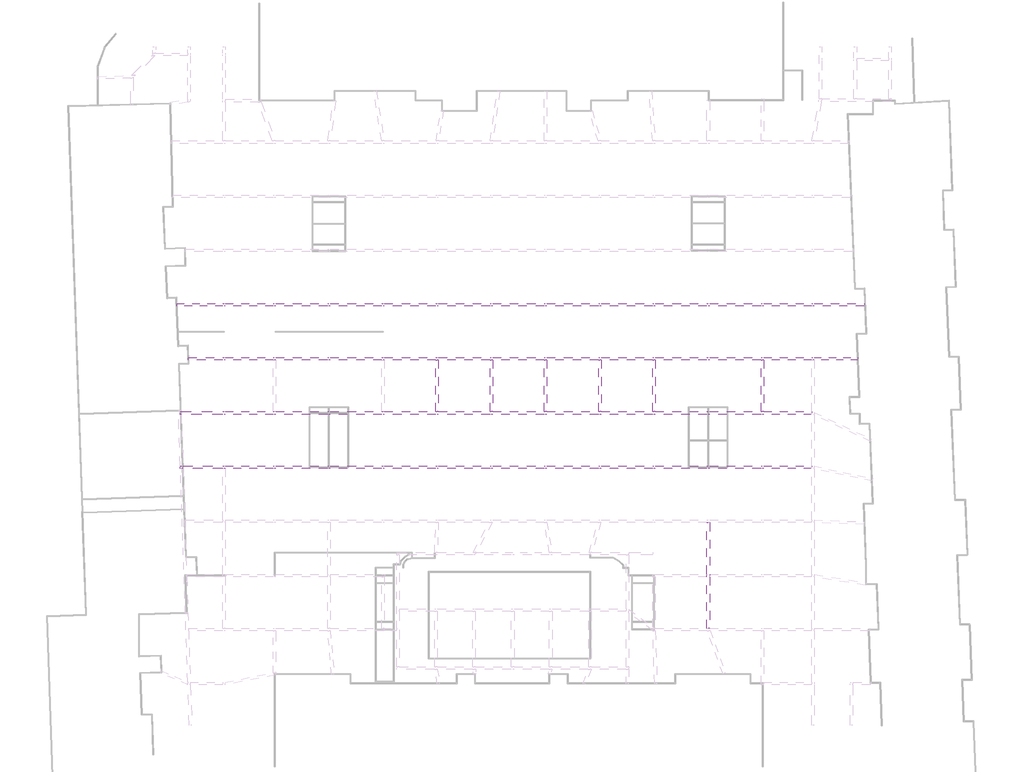
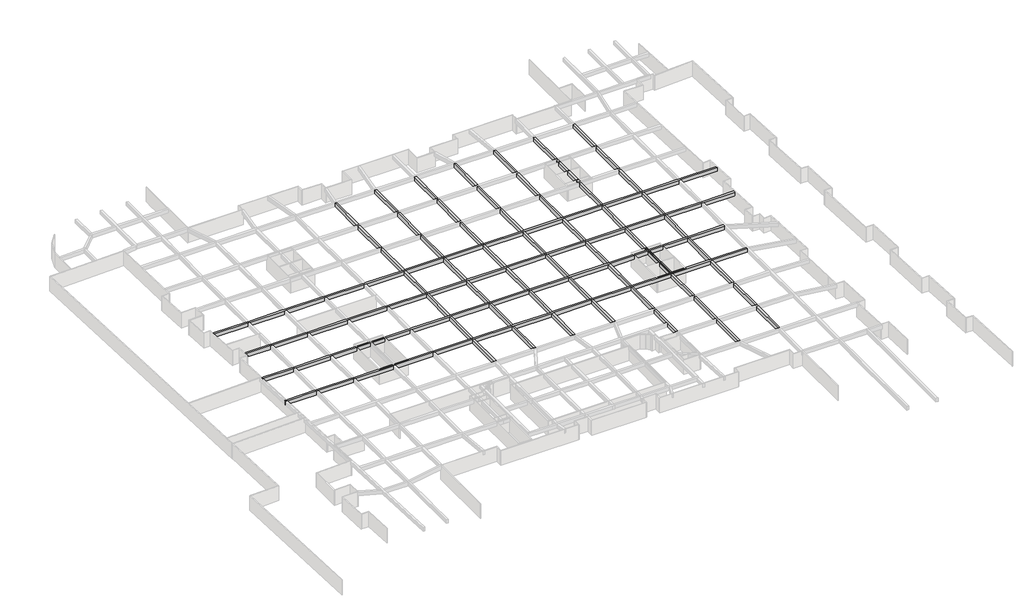
# One storey, part 7 of 8: 11 beams.
"""IFC4 building model written with IfcOpenShell, lengths in millimetres."""

import ifcopenshell
import ifcopenshell.guid

model = None  # the IFC model being written
_history = None  # IfcOwnerHistory: only IFC2X3 demands one
_inside = {}  # id of a spatial element -> (the spatial element, [elements in it])
_under = {}  # id of a project, library or spatial element -> (it, [spatial elements below it])
_declared = {}  # id of a project -> (the project, [libraries it declares])
_typed = {}  # id of a type object -> (the type object, [elements of that type])
_made_of = {}  # id of a material, layer set ... -> (it, [elements and type objects made of it])


def new_model(schema):
    """Start an empty IFC model of exactly this schema.

    Asked for "IFC4X3", IfcOpenShell would pick the latest addendum, in which some entities
    have other attributes; the version numbers below select the first issue.
    IFC2X3 requires an IfcOwnerHistory on every rooted entity: one is made here for all.
    """
    global model, _history
    if schema == "IFC4X3":
        model = ifcopenshell.file(schema_version=(4, 3, 0, 0))
    else:
        model = ifcopenshell.file(schema=schema)
    _inside.clear()
    _under.clear()
    _declared.clear()
    _typed.clear()
    _made_of.clear()
    _history = None
    if model.schema == "IFC2X3":
        org = make("IfcOrganization", Name="unknown")
        user = make(
            "IfcPersonAndOrganization",
            ThePerson=make("IfcPerson", FamilyName="unknown"),
            TheOrganization=org,
        )
        app = make(
            "IfcApplication",
            ApplicationDeveloper=org,
            Version="unknown",
            ApplicationFullName="unknown",
            ApplicationIdentifier="unknown",
        )
        _history = make(
            "IfcOwnerHistory",
            OwningUser=user,
            OwningApplication=app,
            ChangeAction="ADDED",
            CreationDate=0,
        )
    return model


def make(cls, **values):
    """One entity of the class cls with the attributes given. An attribute that is None is left unset."""
    return model.create_entity(
        cls, **{name: value for name, value in values.items() if value is not None}
    )


def rooted(cls, **values):
    """An entity with a GlobalId (a new one), such as an element, a storey or a relation."""
    return make(cls, GlobalId=ifcopenshell.guid.new(), OwnerHistory=_history, **values)


def si_unit(unit_type, name, prefix=None):
    """IfcSIUnit, for example si_unit("LENGTHUNIT", "METRE", prefix="MILLI")."""
    return make("IfcSIUnit", UnitType=unit_type, Prefix=prefix, Name=name)


def assignment(units):
    """IfcUnitAssignment: the units of a project."""
    return None if units is None else make("IfcUnitAssignment", Units=units)


def point(xyz):
    """IfcCartesianPoint."""
    return None if xyz is None else make("IfcCartesianPoint", Coordinates=xyz)


def direction(xyz):
    """IfcDirection."""
    return None if xyz is None else make("IfcDirection", DirectionRatios=xyz)


def frame(location, z_axis=None, x_axis=None):
    """IfcAxis2Placement3D, a coordinate frame: its origin and axes. An axis left out is left unset."""
    return make(
        "IfcAxis2Placement3D",
        Location=point(location),
        Axis=direction(z_axis),
        RefDirection=direction(x_axis),
    )


def origin():
    """The frame at (0, 0, 0) with its axes left unset."""
    return frame((0.0, 0.0, 0.0))


def place(relative_to, where):
    """IfcLocalPlacement: puts the frame where relative to a parent placement (None: the world)."""
    return make(
        "IfcLocalPlacement", PlacementRelTo=relative_to, RelativePlacement=where
    )


def context(
    kind, dimensions, precision=None, world=None, true_north=None, identifier=None
):
    """IfcGeometricRepresentationContext, for example the 3D "Model" context."""
    return make(
        "IfcGeometricRepresentationContext",
        ContextIdentifier=identifier,
        ContextType=kind,
        CoordinateSpaceDimension=dimensions,
        Precision=precision,
        WorldCoordinateSystem=world,
        TrueNorth=true_north,
    )


def project(units=None, contexts=None):
    """IfcProject with its units and contexts."""
    return rooted(
        "IfcProject",
        Name="project",
        RepresentationContexts=contexts,
        UnitsInContext=assignment(units),
    )


def spatial(cls, under=None, at=None, **own):
    """A site, building, storey or space (cls), placed at a placement, below another one or the project."""
    s = rooted(cls, ObjectPlacement=at, **own)
    if under is not None:
        _under.setdefault(under.id(), (under, []))[1].append(s)
    return s


def polyline(points):
    """IfcPolyline through the points."""
    return make("IfcPolyline", Points=[point(p) for p in points])


def outline(outer, holes=None, kind="AREA"):
    """IfcArbitraryClosedProfileDef: a profile drawn as a closed curve; with holes, ...WithVoids."""
    if holes is None:
        return make("IfcArbitraryClosedProfileDef", ProfileType=kind, OuterCurve=outer)
    return make(
        "IfcArbitraryProfileDefWithVoids",
        ProfileType=kind,
        OuterCurve=outer,
        InnerCurves=holes,
    )


def extrude(swept, where, along, depth):
    """IfcExtrudedAreaSolid: the profile swept, set in the frame where, extruded along a direction by depth."""
    return make(
        "IfcExtrudedAreaSolid",
        SweptArea=swept,
        Position=where,
        ExtrudedDirection=direction(along),
        Depth=depth,
    )


def faces_of(points, faces, orient=None, outer=None):
    """IfcFace entities. A face is a list of loops; a loop is a list of indices into points, from 0.

    orient and outer hold one flag for each loop. By default every Orientation is true, the
    first loop of a face is its IfcFaceOuterBound and the others are IfcFaceBound.
    """
    made = []
    for i, loops in enumerate(faces):
        bounds = []
        for j, loop in enumerate(loops):
            is_outer = j == 0 if outer is None else outer[i][j]
            bounds.append(
                make(
                    "IfcFaceOuterBound" if is_outer else "IfcFaceBound",
                    Bound=make("IfcPolyLoop", Polygon=[points[k] for k in loop]),
                    Orientation=True if orient is None else orient[i][j],
                )
            )
        made.append(make("IfcFace", Bounds=bounds))
    return made


def faceted_brep(points, faces, orient=None, outer=None, voids=None):
    """IfcFacetedBrep: a solid bounded by flat faces; with voids (closed shells), ...WithVoids."""
    shared = [point(p) for p in points]
    hull = make("IfcClosedShell", CfsFaces=faces_of(shared, faces, orient, outer))
    if voids is None:
        return make("IfcFacetedBrep", Outer=hull)
    return make(
        "IfcFacetedBrepWithVoids",
        Outer=hull,
        Voids=[
            make(cls, CfsFaces=faces_of(shared, fs, o, b)) for cls, fs, o, b in voids
        ],
    )


def shape(context_of_items, identifier, shape_type, items):
    """IfcShapeRepresentation: the items that make up one representation, for example the "Body"."""
    return make(
        "IfcShapeRepresentation",
        ContextOfItems=context_of_items,
        RepresentationIdentifier=identifier,
        RepresentationType=shape_type,
        Items=items,
    )


def made_of(thing, what):
    """Note that an element or type object is made of a material, layer set ...; save() writes the relation."""
    if what is not None:
        _made_of.setdefault(what.id(), (what, []))[1].append(thing)
    return thing


def element(
    cls,
    number,
    at=None,
    inside=None,
    cuts=None,
    type_object=None,
    material=None,
    context=None,
    identifier="Body",
    shape_type=None,
    held_by="IfcProductDefinitionShape",
    body=None,
    shapes=None,
    **own,
):
    """One element of the class cls, such as IfcWall. Its Tag is "e" and its number.

    at: its placement. inside: the storey or other place that contains it. cuts: it is an
    opening in that element (IfcRelVoidsElement). A single representation is given by context,
    identifier, shape_type and body (its items); several are given by shapes. held_by: the class
    of the entity that holds the representations. save() writes the other relations.
    """
    e = rooted(cls, Tag="e%d" % number, ObjectPlacement=at, **own)
    if body is not None:
        shapes = [shape(context, identifier, shape_type, body)]
    if shapes is not None:
        e.Representation = make(held_by, Representations=shapes)
    if inside is not None:
        _inside.setdefault(inside.id(), (inside, []))[1].append(e)
    if cuts is not None:
        rooted(
            "IfcRelVoidsElement", RelatingBuildingElement=cuts, RelatedOpeningElement=e
        )
    if type_object is not None:
        _typed.setdefault(type_object.id(), (type_object, []))[1].append(e)
    return made_of(e, material)


def aggregate(whole, parts):
    """IfcRelAggregates: a whole, such as a stair, and the parts it consists of."""
    return rooted("IfcRelAggregates", RelatingObject=whole, RelatedObjects=parts)


def save(model, path):
    """Write the relations noted so far, then the file.

    IfcRelAggregates (storeys below a building ...), IfcRelContainedInSpatialStructure (elements
    in a storey), IfcRelDefinesByType, IfcRelAssociatesMaterial and IfcRelDeclares: one each for
    every whole, place, type object, material and project.
    """
    for whole, parts in _under.values():
        aggregate(whole, parts)
    for where, things in _inside.values():
        rooted(
            "IfcRelContainedInSpatialStructure",
            RelatedElements=things,
            RelatingStructure=where,
        )
    for kind, things in _typed.values():
        rooted("IfcRelDefinesByType", RelatedObjects=things, RelatingType=kind)
    for what, things in _made_of.values():
        rooted("IfcRelAssociatesMaterial", RelatedObjects=things, RelatingMaterial=what)
    for by, libraries in _declared.values():
        rooted("IfcRelDeclares", RelatingContext=by, RelatedDefinitions=libraries)
    model.write(path)


model = new_model("IFC4")

# Units and contexts
model_context = context("Model", 3, world=origin())
ifc_project = project(units=[si_unit("LENGTHUNIT", "METRE", prefix="MILLI")], contexts=[model_context])

# Site, building, storey
site = spatial("IfcSite", under=ifc_project)
building = spatial("IfcBuilding", under=site)
storey = spatial("IfcBuildingStorey", under=building, Name="户型图", Elevation=0.0)

# Beams
placement = place(None, origin())
element("IfcBeam", 1, ObjectType="混凝土 - 矩形梁 : KL_beam", at=placement, inside=storey, context=model_context, shape_type="Brep", body=[
    faceted_brep([(776034.6775785, -933866.0928676, 3300.0), (776034.6775785, -934266.0928676, 3300.0), (776034.6775785, -934266.0928676, 2500.0), (776034.6775785, -933866.0928676, 2500.0), (669471.6775785, -933866.0928676, 3300.0), (669471.6775785, -933866.0928676, 2500.0), (669471.6775785, -934266.0928676, 2500.0), (669471.6775785, -934266.0928676, 3300.0), (768294.1555611, -933866.0928676, 3300.0), (767894.1555611, -933866.0928676, 3300.0), (760462.0478253, -933866.0928676, 3300.0), (760062.0478253, -933866.0928676, 3300.0), (752074.1555611, -933866.0928676, 3300.0), (751674.1555611, -933866.0928676, 3300.0), (743652.0478253, -933866.0928676, 3300.0), (743252.0478253, -933866.0928676, 3300.0), (735261.5831818, -933866.0928676, 3300.0), (734861.5831818, -933866.0928676, 3300.0), (726824.1555611, -933866.0928676, 3300.0), (726424.1555611, -933866.0928676, 3300.0), (718446.3042159, -933866.0928676, 3300.0), (718046.3042159, -933866.0928676, 3300.0), (710046.3042159, -933866.0928676, 3300.0), (709646.3042159, -933866.0928676, 3300.0), (701672.0478253, -933866.0928676, 3300.0), (701272.0478253, -933866.0928676, 3300.0), (693274.1555611, -933866.0928676, 3300.0), (692874.1555611, -933866.0928676, 3300.0), (684802.0478253, -933866.0928676, 3300.0), (684402.0478253, -933866.0928676, 3300.0), (677027.1185384, -933866.0928676, 3300.0), (676627.1185384, -933866.0928676, 3300.0), (676627.1185384, -934266.0928676, 3300.0), (677027.1185384, -934266.0928676, 3300.0), (684402.0478253, -934266.0928676, 3300.0), (684802.0478253, -934266.0928676, 3300.0), (692874.1555611, -934266.0928676, 3300.0), (693274.1555611, -934266.0928676, 3300.0), (701272.0478253, -934266.0928676, 3300.0), (701672.0478253, -934266.0928676, 3300.0), (709646.3042159, -934266.0928676, 3300.0), (710046.3042159, -934266.0928676, 3300.0), (718046.3042159, -934266.0928676, 3300.0), (718446.3042159, -934266.0928676, 3300.0), (726424.1555611, -934266.0928676, 3300.0), (726824.1555611, -934266.0928676, 3300.0), (734861.5831818, -934266.0928676, 3300.0), (735261.5831818, -934266.0928676, 3300.0), (743252.0478253, -934266.0928676, 3300.0), (743652.0478253, -934266.0928676, 3300.0), (751674.1555611, -934266.0928676, 3300.0), (752074.1555611, -934266.0928676, 3300.0), (760062.0478253, -934266.0928676, 3300.0), (760462.0478253, -934266.0928676, 3300.0), (767894.1555611, -934266.0928676, 3300.0), (768294.1555611, -934266.0928676, 3300.0), (676627.1185384, -934266.0928676, 2500.0), (677027.1185384, -934266.0928676, 2500.0), (684402.0478253, -934266.0928676, 2500.0), (684802.0478253, -934266.0928676, 2500.0), (692874.1555611, -934266.0928676, 2500.0), (693274.1555611, -934266.0928676, 2500.0), (701272.0478253, -934266.0928676, 2500.0), (701672.0478253, -934266.0928676, 2500.0), (709646.3042159, -934266.0928676, 2500.0), (710046.3042159, -934266.0928676, 2500.0), (718046.3042159, -934266.0928676, 2500.0), (718446.3042159, -934266.0928676, 2500.0), (726424.1555611, -934266.0928676, 2500.0), (726824.1555611, -934266.0928676, 2500.0), (734861.5831818, -934266.0928676, 2500.0), (735261.5831818, -934266.0928676, 2500.0), (743252.0478253, -934266.0928676, 2500.0), (743652.0478253, -934266.0928676, 2500.0), (751674.1555611, -934266.0928676, 2500.0), (752074.1555611, -934266.0928676, 2500.0), (760062.0478253, -934266.0928676, 2500.0), (760462.0478253, -934266.0928676, 2500.0), (767894.1555611, -934266.0928676, 2500.0), (768294.1555611, -934266.0928676, 2500.0), (676627.1185384, -933866.0928676, 2500.0), (677027.1185384, -933866.0928676, 2500.0), (684402.0478253, -933866.0928676, 2500.0), (684802.0478253, -933866.0928676, 2500.0), (692874.1555611, -933866.0928676, 2500.0), (693274.1555611, -933866.0928676, 2500.0), (701272.0478253, -933866.0928676, 2500.0), (701672.0478253, -933866.0928676, 2500.0), (709646.3042159, -933866.0928676, 2500.0), (710046.3042159, -933866.0928676, 2500.0), (718046.3042159, -933866.0928676, 2500.0), (718446.3042159, -933866.0928676, 2500.0), (726424.1555611, -933866.0928676, 2500.0), (726824.1555611, -933866.0928676, 2500.0), (734861.5831818, -933866.0928676, 2500.0), (735261.5831818, -933866.0928676, 2500.0), (743252.0478253, -933866.0928676, 2500.0), (743652.0478253, -933866.0928676, 2500.0), (751674.1555611, -933866.0928676, 2500.0), (752074.1555611, -933866.0928676, 2500.0), (760062.0478253, -933866.0928676, 2500.0), (760462.0478253, -933866.0928676, 2500.0), (767894.1555611, -933866.0928676, 2500.0), (768294.1555611, -933866.0928676, 2500.0)], [[[0, 1, 2, 3]], [[4, 5, 6, 7]], [[1, 0, 8, 9, 10, 11, 12, 13, 14, 15, 16, 17, 18, 19, 20, 21, 22, 23, 24, 25, 26, 27, 28, 29, 30, 31, 4, 7, 32, 33, 34, 35, 36, 37, 38, 39, 40, 41, 42, 43, 44, 45, 46, 47, 48, 49, 50, 51, 52, 53, 54, 55]], [[2, 1, 55, 54, 53, 52, 51, 50, 49, 48, 47, 46, 45, 44, 43, 42, 41, 40, 39, 38, 37, 36, 35, 34, 33, 32, 7, 6, 56, 57, 58, 59, 60, 61, 62, 63, 64, 65, 66, 67, 68, 69, 70, 71, 72, 73, 74, 75, 76, 77, 78, 79]], [[3, 2, 79, 78, 77, 76, 75, 74, 73, 72, 71, 70, 69, 68, 67, 66, 65, 64, 63, 62, 61, 60, 59, 58, 57, 56, 6, 5, 80, 81, 82, 83, 84, 85, 86, 87, 88, 89, 90, 91, 92, 93, 94, 95, 96, 97, 98, 99, 100, 101, 102, 103]], [[0, 3, 103, 102, 101, 100, 99, 98, 97, 96, 95, 94, 93, 92, 91, 90, 89, 88, 87, 86, 85, 84, 83, 82, 81, 80, 5, 4, 31, 30, 29, 28, 27, 26, 25, 24, 23, 22, 21, 20, 19, 18, 17, 16, 15, 14, 13, 12, 11, 10, 9, 8]]]),
])
element("IfcBeam", 2, ObjectType="混凝土 - 矩形梁 : KL_beam", at=placement, inside=storey, context=model_context, shape_type="Brep", body=[
    faceted_brep([(775074.5999957, -942255.576527, 3300.0), (775074.5999957, -942655.576527, 3300.0), (775074.5999957, -942655.576527, 2500.0), (775074.5999957, -942255.576527, 2500.0), (671274.5999957, -942255.576527, 3300.0), (671274.5999957, -942255.576527, 2500.0), (671274.5999957, -942655.576527, 2500.0), (671274.5999957, -942655.576527, 3300.0), (768294.1555611, -942255.576527, 3300.0), (767894.1555611, -942255.576527, 3300.0), (760462.0478253, -942255.576527, 3300.0), (760062.0478253, -942255.576527, 3300.0), (752074.1555611, -942255.576527, 3300.0), (751674.1555611, -942255.576527, 3300.0), (743652.0478253, -942255.576527, 3300.0), (743252.0478253, -942255.576527, 3300.0), (735261.5831818, -942255.576527, 3300.0), (734861.5831818, -942255.576527, 3300.0), (726824.1555611, -942255.576527, 3300.0), (726424.1555611, -942255.576527, 3300.0), (718446.3042159, -942255.576527, 3300.0), (718046.3042159, -942255.576527, 3300.0), (710046.3042159, -942255.576527, 3300.0), (709646.3042159, -942255.576527, 3300.0), (701672.0478253, -942255.576527, 3300.0), (701272.0478253, -942255.576527, 3300.0), (693274.1555611, -942255.576527, 3300.0), (692874.1555611, -942255.576527, 3300.0), (684802.0478253, -942255.576527, 3300.0), (684402.0478253, -942255.576527, 3300.0), (677027.1185384, -942255.576527, 3300.0), (676627.1185384, -942255.576527, 3300.0), (676627.1185384, -942655.576527, 3300.0), (677027.1185384, -942655.576527, 3300.0), (684402.0478253, -942655.576527, 3300.0), (684802.0478253, -942655.576527, 3300.0), (692874.1555611, -942655.576527, 3300.0), (693274.1555611, -942655.576527, 3300.0), (701272.0478253, -942655.576527, 3300.0), (701672.0478253, -942655.576527, 3300.0), (709646.3042159, -942655.576527, 3300.0), (710046.3042159, -942655.576527, 3300.0), (718046.3042159, -942655.576527, 3300.0), (718446.3042159, -942655.576527, 3300.0), (726424.1555611, -942655.576527, 3300.0), (726824.1555611, -942655.576527, 3300.0), (734861.5831818, -942655.576527, 3300.0), (735261.5831818, -942655.576527, 3300.0), (743252.0478253, -942655.576527, 3300.0), (743652.0478253, -942655.576527, 3300.0), (751674.1555611, -942655.576527, 3300.0), (752074.1555611, -942655.576527, 3300.0), (760062.0478253, -942655.576527, 3300.0), (760462.0478253, -942655.576527, 3300.0), (767894.1555611, -942655.576527, 3300.0), (768294.1555611, -942655.576527, 3300.0), (676627.1185384, -942655.576527, 2500.0), (677027.1185384, -942655.576527, 2500.0), (684402.0478253, -942655.576527, 2500.0), (684802.0478253, -942655.576527, 2500.0), (692874.1555611, -942655.576527, 2500.0), (693274.1555611, -942655.576527, 2500.0), (701272.0478253, -942655.576527, 2500.0), (701672.0478253, -942655.576527, 2500.0), (709646.3042159, -942655.576527, 2500.0), (710046.3042159, -942655.576527, 2500.0), (718046.3042159, -942655.576527, 2500.0), (718446.3042159, -942655.576527, 2500.0), (726424.1555611, -942655.576527, 2500.0), (726824.1555611, -942655.576527, 2500.0), (734861.5831818, -942655.576527, 2500.0), (735261.5831818, -942655.576527, 2500.0), (743252.0478253, -942655.576527, 2500.0), (743652.0478253, -942655.576527, 2500.0), (751674.1555611, -942655.576527, 2500.0), (752074.1555611, -942655.576527, 2500.0), (760062.0478253, -942655.576527, 2500.0), (760462.0478253, -942655.576527, 2500.0), (767894.1555611, -942655.576527, 2500.0), (768294.1555611, -942655.576527, 2500.0), (676627.1185384, -942255.576527, 2500.0), (677027.1185384, -942255.576527, 2500.0), (684402.0478253, -942255.576527, 2500.0), (684802.0478253, -942255.576527, 2500.0), (692874.1555611, -942255.576527, 2500.0), (693274.1555611, -942255.576527, 2500.0), (701272.0478253, -942255.576527, 2500.0), (701672.0478253, -942255.576527, 2500.0), (709646.3042159, -942255.576527, 2500.0), (710046.3042159, -942255.576527, 2500.0), (718046.3042159, -942255.576527, 2500.0), (718446.3042159, -942255.576527, 2500.0), (726424.1555611, -942255.576527, 2500.0), (726824.1555611, -942255.576527, 2500.0), (734861.5831818, -942255.576527, 2500.0), (735261.5831818, -942255.576527, 2500.0), (743252.0478253, -942255.576527, 2500.0), (743652.0478253, -942255.576527, 2500.0), (751674.1555611, -942255.576527, 2500.0), (752074.1555611, -942255.576527, 2500.0), (760062.0478253, -942255.576527, 2500.0), (760462.0478253, -942255.576527, 2500.0), (767894.1555611, -942255.576527, 2500.0), (768294.1555611, -942255.576527, 2500.0)], [[[0, 1, 2, 3]], [[4, 5, 6, 7]], [[1, 0, 8, 9, 10, 11, 12, 13, 14, 15, 16, 17, 18, 19, 20, 21, 22, 23, 24, 25, 26, 27, 28, 29, 30, 31, 4, 7, 32, 33, 34, 35, 36, 37, 38, 39, 40, 41, 42, 43, 44, 45, 46, 47, 48, 49, 50, 51, 52, 53, 54, 55]], [[2, 1, 55, 54, 53, 52, 51, 50, 49, 48, 47, 46, 45, 44, 43, 42, 41, 40, 39, 38, 37, 36, 35, 34, 33, 32, 7, 6, 56, 57, 58, 59, 60, 61, 62, 63, 64, 65, 66, 67, 68, 69, 70, 71, 72, 73, 74, 75, 76, 77, 78, 79]], [[3, 2, 79, 78, 77, 76, 75, 74, 73, 72, 71, 70, 69, 68, 67, 66, 65, 64, 63, 62, 61, 60, 59, 58, 57, 56, 6, 5, 80, 81, 82, 83, 84, 85, 86, 87, 88, 89, 90, 91, 92, 93, 94, 95, 96, 97, 98, 99, 100, 101, 102, 103]], [[0, 3, 103, 102, 101, 100, 99, 98, 97, 96, 95, 94, 93, 92, 91, 90, 89, 88, 87, 86, 85, 84, 83, 82, 81, 80, 5, 4, 31, 30, 29, 28, 27, 26, 25, 24, 23, 22, 21, 20, 19, 18, 17, 16, 15, 14, 13, 12, 11, 10, 9, 8]]]),
])
element("IfcBeam", 3, ObjectType="混凝土 - 矩形梁 : KL_beam", at=placement, inside=storey, context=model_context, shape_type="Brep", body=[
    faceted_brep([(670029.8295359, -950666.0928676, 3300.0), (670029.8295359, -950666.0928676, 2500.0), (670029.8295359, -951066.0928676, 2500.0), (670029.8295359, -951066.0928676, 3300.0), (670141.6640504, -951066.0928676, 3300.0), (676627.1185384, -951066.0928676, 3300.0), (677027.1185384, -951066.0928676, 3300.0), (684402.0478253, -951066.0928676, 3300.0), (684802.0478253, -951066.0928676, 3300.0), (692874.1555611, -951066.0928676, 3300.0), (693274.1555611, -951066.0928676, 3300.0), (701272.0478253, -951066.0928676, 3300.0), (701672.0478253, -951066.0928676, 3300.0), (709646.3042159, -951066.0928676, 3300.0), (710046.3042159, -951066.0928676, 3300.0), (718046.3042159, -951066.0928676, 3300.0), (718446.3042159, -951066.0928676, 3300.0), (726424.1555611, -951066.0928676, 3300.0), (726824.1555611, -951066.0928676, 3300.0), (734861.5831818, -951066.0928676, 3300.0), (735261.5831818, -951066.0928676, 3300.0), (743252.0478253, -951066.0928676, 3300.0), (743652.0478253, -951066.0928676, 3300.0), (751674.1555611, -951066.0928676, 3300.0), (752074.1555611, -951066.0928676, 3300.0), (760062.0478253, -951066.0928676, 3300.0), (760462.0478253, -951066.0928676, 3300.0), (767894.1555611, -951066.0928676, 3300.0), (767894.1555611, -950666.0928676, 3300.0), (760462.0478253, -950666.0928676, 3300.0), (760062.0478253, -950666.0928676, 3300.0), (752074.1555611, -950666.0928676, 3300.0), (751674.1555611, -950666.0928676, 3300.0), (743652.0478253, -950666.0928676, 3300.0), (743252.0478253, -950666.0928676, 3300.0), (735261.5831818, -950666.0928676, 3300.0), (734861.5831818, -950666.0928676, 3300.0), (726824.1555611, -950666.0928676, 3300.0), (726424.1555611, -950666.0928676, 3300.0), (718446.3042159, -950666.0928676, 3300.0), (718046.3042159, -950666.0928676, 3300.0), (710046.3042159, -950666.0928676, 3300.0), (709646.3042159, -950666.0928676, 3300.0), (701672.0478253, -950666.0928676, 3300.0), (701272.0478253, -950666.0928676, 3300.0), (693274.1555611, -950666.0928676, 3300.0), (692874.1555611, -950666.0928676, 3300.0), (684802.0478253, -950666.0928676, 3300.0), (684402.0478253, -950666.0928676, 3300.0), (677027.1185384, -950666.0928676, 3300.0), (676627.1185384, -950666.0928676, 3300.0), (670127.6957426, -950666.0928676, 3300.0), (670141.6640504, -951066.0928676, 2500.0), (676627.1185384, -951066.0928676, 2500.0), (677027.1185384, -951066.0928676, 2500.0), (684402.0478253, -951066.0928676, 2500.0), (684802.0478253, -951066.0928676, 2500.0), (692874.1555611, -951066.0928676, 2500.0), (693274.1555611, -951066.0928676, 2500.0), (701272.0478253, -951066.0928676, 2500.0), (701672.0478253, -951066.0928676, 2500.0), (709646.3042159, -951066.0928676, 2500.0), (710046.3042159, -951066.0928676, 2500.0), (718046.3042159, -951066.0928676, 2500.0), (718446.3042159, -951066.0928676, 2500.0), (726424.1555611, -951066.0928676, 2500.0), (726824.1555611, -951066.0928676, 2500.0), (734861.5831818, -951066.0928676, 2500.0), (735261.5831818, -951066.0928676, 2500.0), (743252.0478253, -951066.0928676, 2500.0), (743652.0478253, -951066.0928676, 2500.0), (751674.1555611, -951066.0928676, 2500.0), (752074.1555611, -951066.0928676, 2500.0), (760062.0478253, -951066.0928676, 2500.0), (760462.0478253, -951066.0928676, 2500.0), (767894.1555611, -951066.0928676, 2500.0), (670127.6957426, -950666.0928676, 2500.0), (676627.1185384, -950666.0928676, 2500.0), (677027.1185384, -950666.0928676, 2500.0), (684402.0478253, -950666.0928676, 2500.0), (684802.0478253, -950666.0928676, 2500.0), (692874.1555611, -950666.0928676, 2500.0), (693274.1555611, -950666.0928676, 2500.0), (701272.0478253, -950666.0928676, 2500.0), (701672.0478253, -950666.0928676, 2500.0), (709646.3042159, -950666.0928676, 2500.0), (710046.3042159, -950666.0928676, 2500.0), (718046.3042159, -950666.0928676, 2500.0), (718446.3042159, -950666.0928676, 2500.0), (726424.1555611, -950666.0928676, 2500.0), (726824.1555611, -950666.0928676, 2500.0), (734861.5831818, -950666.0928676, 2500.0), (735261.5831818, -950666.0928676, 2500.0), (743252.0478253, -950666.0928676, 2500.0), (743652.0478253, -950666.0928676, 2500.0), (751674.1555611, -950666.0928676, 2500.0), (752074.1555611, -950666.0928676, 2500.0), (760062.0478253, -950666.0928676, 2500.0), (760462.0478253, -950666.0928676, 2500.0), (767894.1555611, -950666.0928676, 2500.0)], [[[0, 1, 2, 3]], [[0, 3, 4, 5, 6, 7, 8, 9, 10, 11, 12, 13, 14, 15, 16, 17, 18, 19, 20, 21, 22, 23, 24, 25, 26, 27, 28, 29, 30, 31, 32, 33, 34, 35, 36, 37, 38, 39, 40, 41, 42, 43, 44, 45, 46, 47, 48, 49, 50, 51]], [[3, 2, 52, 53, 54, 55, 56, 57, 58, 59, 60, 61, 62, 63, 64, 65, 66, 67, 68, 69, 70, 71, 72, 73, 74, 75, 27, 26, 25, 24, 23, 22, 21, 20, 19, 18, 17, 16, 15, 14, 13, 12, 11, 10, 9, 8, 7, 6, 5, 4]], [[2, 1, 76, 77, 78, 79, 80, 81, 82, 83, 84, 85, 86, 87, 88, 89, 90, 91, 92, 93, 94, 95, 96, 97, 98, 99, 75, 74, 73, 72, 71, 70, 69, 68, 67, 66, 65, 64, 63, 62, 61, 60, 59, 58, 57, 56, 55, 54, 53, 52]], [[1, 0, 51, 50, 49, 48, 47, 46, 45, 44, 43, 42, 41, 40, 39, 38, 37, 36, 35, 34, 33, 32, 31, 30, 29, 28, 99, 98, 97, 96, 95, 94, 93, 92, 91, 90, 89, 88, 87, 86, 85, 84, 83, 82, 81, 80, 79, 78, 77, 76]], [[28, 27, 75, 99]]]),
])
element("IfcBeam", 4, ObjectType="混凝土 - 矩形梁 : KL_beam", at=placement, inside=storey, context=model_context, shape_type="Brep", body=[
    faceted_brep([(670034.250673, -959062.643437, 3300.0), (670034.250673, -959462.643437, 3300.0), (670434.4944908, -959462.643437, 3300.0), (676627.1185384, -959462.643437, 3300.0), (677027.1185384, -959462.643437, 3300.0), (684402.0478253, -959462.643437, 3300.0), (684802.0478253, -959462.643437, 3300.0), (692874.1555611, -959462.643437, 3300.0), (693274.1555611, -959462.643437, 3300.0), (701272.0478253, -959462.643437, 3300.0), (701672.0478253, -959462.643437, 3300.0), (709646.3042159, -959462.643437, 3300.0), (710046.3042159, -959462.643437, 3300.0), (718046.3042159, -959462.643437, 3300.0), (718446.3042159, -959462.643437, 3300.0), (726424.1555611, -959462.643437, 3300.0), (726824.1555611, -959462.643437, 3300.0), (734861.5831818, -959462.643437, 3300.0), (735261.5831818, -959462.643437, 3300.0), (743252.0478253, -959462.643437, 3300.0), (743652.0478253, -959462.643437, 3300.0), (751674.1555611, -959462.643437, 3300.0), (752074.1555611, -959462.643437, 3300.0), (760062.0478253, -959462.643437, 3300.0), (760462.0478253, -959462.643437, 3300.0), (767894.1555611, -959462.643437, 3300.0), (767894.1555611, -959062.643437, 3300.0), (760462.0478253, -959062.643437, 3300.0), (760062.0478253, -959062.643437, 3300.0), (752074.1555611, -959062.643437, 3300.0), (751674.1555611, -959062.643437, 3300.0), (743652.0478253, -959062.643437, 3300.0), (743252.0478253, -959062.643437, 3300.0), (735261.5831818, -959062.643437, 3300.0), (734861.5831818, -959062.643437, 3300.0), (726824.1555611, -959062.643437, 3300.0), (726424.1555611, -959062.643437, 3300.0), (718446.3042159, -959062.643437, 3300.0), (718046.3042159, -959062.643437, 3300.0), (710046.3042159, -959062.643437, 3300.0), (709646.3042159, -959062.643437, 3300.0), (701672.0478253, -959062.643437, 3300.0), (701272.0478253, -959062.643437, 3300.0), (693274.1555611, -959062.643437, 3300.0), (692874.1555611, -959062.643437, 3300.0), (684802.0478253, -959062.643437, 3300.0), (684402.0478253, -959062.643437, 3300.0), (677027.1185384, -959062.643437, 3300.0), (676627.1185384, -959062.643437, 3300.0), (670420.9097495, -959062.643437, 3300.0), (670034.250673, -959462.643437, 2500.0), (670434.4944908, -959462.643437, 2500.0), (676627.1185384, -959462.643437, 2500.0), (677027.1185384, -959462.643437, 2500.0), (684402.0478253, -959462.643437, 2500.0), (684802.0478253, -959462.643437, 2500.0), (692874.1555611, -959462.643437, 2500.0), (693274.1555611, -959462.643437, 2500.0), (701272.0478253, -959462.643437, 2500.0), (701672.0478253, -959462.643437, 2500.0), (709646.3042159, -959462.643437, 2500.0), (710046.3042159, -959462.643437, 2500.0), (718046.3042159, -959462.643437, 2500.0), (718446.3042159, -959462.643437, 2500.0), (726424.1555611, -959462.643437, 2500.0), (726824.1555611, -959462.643437, 2500.0), (734861.5831818, -959462.643437, 2500.0), (735261.5831818, -959462.643437, 2500.0), (743252.0478253, -959462.643437, 2500.0), (743652.0478253, -959462.643437, 2500.0), (751674.1555611, -959462.643437, 2500.0), (752074.1555611, -959462.643437, 2500.0), (760062.0478253, -959462.643437, 2500.0), (760462.0478253, -959462.643437, 2500.0), (767894.1555611, -959462.643437, 2500.0), (670034.250673, -959062.643437, 2500.0), (670420.9097495, -959062.643437, 2500.0), (676627.1185384, -959062.643437, 2500.0), (677027.1185384, -959062.643437, 2500.0), (684402.0478253, -959062.643437, 2500.0), (684802.0478253, -959062.643437, 2500.0), (692874.1555611, -959062.643437, 2500.0), (693274.1555611, -959062.643437, 2500.0), (701272.0478253, -959062.643437, 2500.0), (701672.0478253, -959062.643437, 2500.0), (709646.3042159, -959062.643437, 2500.0), (710046.3042159, -959062.643437, 2500.0), (718046.3042159, -959062.643437, 2500.0), (718446.3042159, -959062.643437, 2500.0), (726424.1555611, -959062.643437, 2500.0), (726824.1555611, -959062.643437, 2500.0), (734861.5831818, -959062.643437, 2500.0), (735261.5831818, -959062.643437, 2500.0), (743252.0478253, -959062.643437, 2500.0), (743652.0478253, -959062.643437, 2500.0), (751674.1555611, -959062.643437, 2500.0), (752074.1555611, -959062.643437, 2500.0), (760062.0478253, -959062.643437, 2500.0), (760462.0478253, -959062.643437, 2500.0), (767894.1555611, -959062.643437, 2500.0)], [[[0, 1, 2, 3, 4, 5, 6, 7, 8, 9, 10, 11, 12, 13, 14, 15, 16, 17, 18, 19, 20, 21, 22, 23, 24, 25, 26, 27, 28, 29, 30, 31, 32, 33, 34, 35, 36, 37, 38, 39, 40, 41, 42, 43, 44, 45, 46, 47, 48, 49]], [[1, 50, 51, 52, 53, 54, 55, 56, 57, 58, 59, 60, 61, 62, 63, 64, 65, 66, 67, 68, 69, 70, 71, 72, 73, 74, 25, 24, 23, 22, 21, 20, 19, 18, 17, 16, 15, 14, 13, 12, 11, 10, 9, 8, 7, 6, 5, 4, 3, 2]], [[50, 75, 76, 77, 78, 79, 80, 81, 82, 83, 84, 85, 86, 87, 88, 89, 90, 91, 92, 93, 94, 95, 96, 97, 98, 99, 74, 73, 72, 71, 70, 69, 68, 67, 66, 65, 64, 63, 62, 61, 60, 59, 58, 57, 56, 55, 54, 53, 52, 51]], [[75, 0, 49, 48, 47, 46, 45, 44, 43, 42, 41, 40, 39, 38, 37, 36, 35, 34, 33, 32, 31, 30, 29, 28, 27, 26, 99, 98, 97, 96, 95, 94, 93, 92, 91, 90, 89, 88, 87, 86, 85, 84, 83, 82, 81, 80, 79, 78, 77, 76]], [[26, 25, 74, 99]], [[0, 75, 50, 1]]]),
])
element("IfcBeam", 5, ObjectType="混凝土 - 矩形梁 : KL_beam", at=placement, inside=storey, context=model_context, shape_type="SweptSolid", body=[
    extrude(outline(polyline([(709646.3042159, -909063.5696638), (710046.3042159, -909063.5696638), (710046.3042159, -917066.0928676), (709646.3042159, -917066.0928676), (709646.3042159, -909063.5696638)])), frame((0.0, 0.0, 2500.0), z_axis=(0.0, 0.0, 1.0), x_axis=(1.0, 0.0, 0.0)), (0.0, 0.0, 1.0), 800.0),
    extrude(outline(polyline([(710046.3042159, -967466.0928676), (709646.3042159, -967466.0928676), (709646.3042159, -959462.643437), (710046.3042159, -959462.643437), (710046.3042159, -967466.0928676)])), frame((0.0, 0.0, 2500.0), z_axis=(0.0, 0.0, 1.0), x_axis=(1.0, 0.0, 0.0)), (0.0, 0.0, 1.0), 800.0),
    extrude(outline(polyline([(709646.3042159, -917466.0928676), (710046.3042159, -917466.0928676), (710046.3042159, -925466.8334343), (709646.3042159, -925466.8334343), (709646.3042159, -917466.0928676)])), frame((0.0, 0.0, 2500.0), z_axis=(0.0, 0.0, 1.0), x_axis=(1.0, 0.0, 0.0)), (0.0, 0.0, 1.0), 800.0),
    extrude(outline(polyline([(709646.3042159, -925866.8334343), (710046.3042159, -925866.8334343), (710046.3042159, -933866.0928676), (709646.3042159, -933866.0928676), (709646.3042159, -925866.8334343)])), frame((0.0, 0.0, 2500.0), z_axis=(0.0, 0.0, 1.0), x_axis=(1.0, 0.0, 0.0)), (0.0, 0.0, 1.0), 800.0),
    extrude(outline(polyline([(709646.3042159, -934266.0928676), (710046.3042159, -934266.0928676), (710046.3042159, -942255.576527), (709646.3042159, -942255.576527), (709646.3042159, -934266.0928676)])), frame((0.0, 0.0, 2500.0), z_axis=(0.0, 0.0, 1.0), x_axis=(1.0, 0.0, 0.0)), (0.0, 0.0, 1.0), 800.0),
    extrude(outline(polyline([(709646.3042159, -942655.576527), (710046.3042159, -942655.576527), (710046.3042159, -950666.0928676), (709646.3042159, -950666.0928676), (709646.3042159, -942655.576527)])), frame((0.0, 0.0, 2500.0), z_axis=(0.0, 0.0, 1.0), x_axis=(1.0, 0.0, 0.0)), (0.0, 0.0, 1.0), 800.0),
    extrude(outline(polyline([(709646.3042159, -951066.0928676), (710046.3042159, -951066.0928676), (710046.3042159, -959062.643437), (709646.3042159, -959062.643437), (709646.3042159, -951066.0928676)])), frame((0.0, 0.0, 2500.0), z_axis=(0.0, 0.0, 1.0), x_axis=(1.0, 0.0, 0.0)), (0.0, 0.0, 1.0), 800.0),
])
element("IfcBeam", 6, ObjectType="混凝土 - 矩形梁 : KL_beam", at=placement, inside=storey, context=model_context, shape_type="SweptSolid", body=[
    extrude(outline(polyline([(718446.3042159, -967466.0928676), (718046.3042159, -967466.0928676), (718046.3042159, -959462.643437), (718446.3042159, -959462.643437), (718446.3042159, -967466.0928676)])), frame((0.0, 0.0, 2500.0), z_axis=(0.0, 0.0, 1.0), x_axis=(1.0, 0.0, 0.0)), (0.0, 0.0, 1.0), 800.0),
    extrude(outline(polyline([(718046.3042159, -909063.5696638), (718446.3042159, -909063.5696638), (718446.3042159, -917066.0928676), (718046.3042159, -917066.0928676), (718046.3042159, -909063.5696638)])), frame((0.0, 0.0, 2500.0), z_axis=(0.0, 0.0, 1.0), x_axis=(1.0, 0.0, 0.0)), (0.0, 0.0, 1.0), 800.0),
    extrude(outline(polyline([(718046.3042159, -917466.0928676), (718446.3042159, -917466.0928676), (718446.3042159, -925466.8334343), (718046.3042159, -925466.8334343), (718046.3042159, -917466.0928676)])), frame((0.0, 0.0, 2500.0), z_axis=(0.0, 0.0, 1.0), x_axis=(1.0, 0.0, 0.0)), (0.0, 0.0, 1.0), 800.0),
    extrude(outline(polyline([(718046.3042159, -925866.8334343), (718446.3042159, -925866.8334343), (718446.3042159, -933866.0928676), (718046.3042159, -933866.0928676), (718046.3042159, -925866.8334343)])), frame((0.0, 0.0, 2500.0), z_axis=(0.0, 0.0, 1.0), x_axis=(1.0, 0.0, 0.0)), (0.0, 0.0, 1.0), 800.0),
    extrude(outline(polyline([(718046.3042159, -934266.0928676), (718446.3042159, -934266.0928676), (718446.3042159, -942255.576527), (718046.3042159, -942255.576527), (718046.3042159, -934266.0928676)])), frame((0.0, 0.0, 2500.0), z_axis=(0.0, 0.0, 1.0), x_axis=(1.0, 0.0, 0.0)), (0.0, 0.0, 1.0), 800.0),
    extrude(outline(polyline([(718046.3042159, -942655.576527), (718446.3042159, -942655.576527), (718446.3042159, -950666.0928676), (718046.3042159, -950666.0928676), (718046.3042159, -942655.576527)])), frame((0.0, 0.0, 2500.0), z_axis=(0.0, 0.0, 1.0), x_axis=(1.0, 0.0, 0.0)), (0.0, 0.0, 1.0), 800.0),
    extrude(outline(polyline([(718046.3042159, -951066.0928676), (718446.3042159, -951066.0928676), (718446.3042159, -959062.643437), (718046.3042159, -959062.643437), (718046.3042159, -951066.0928676)])), frame((0.0, 0.0, 2500.0), z_axis=(0.0, 0.0, 1.0), x_axis=(1.0, 0.0, 0.0)), (0.0, 0.0, 1.0), 800.0),
])
element("IfcBeam", 7, ObjectType="混凝土 - 矩形梁 : KL_beam", at=placement, inside=storey, context=model_context, shape_type="SweptSolid", body=[
    extrude(outline(polyline([(726424.1555611, -909063.5696638), (726824.1555611, -909063.5696638), (726824.1555611, -917066.0928676), (726424.1555611, -917066.0928676), (726424.1555611, -909063.5696638)])), frame((0.0, 0.0, 2500.0), z_axis=(0.0, 0.0, 1.0), x_axis=(1.0, 0.0, 0.0)), (0.0, 0.0, 1.0), 800.0),
    extrude(outline(polyline([(726824.1555611, -967466.0928676), (726424.1555611, -967466.0928676), (726424.1555611, -959462.643437), (726824.1555611, -959462.643437), (726824.1555611, -967466.0928676)])), frame((0.0, 0.0, 2500.0), z_axis=(0.0, 0.0, 1.0), x_axis=(1.0, 0.0, 0.0)), (0.0, 0.0, 1.0), 800.0),
    extrude(outline(polyline([(726424.1555611, -917466.0928676), (726824.1555611, -917466.0928676), (726824.1555611, -925466.8334343), (726424.1555611, -925466.8334343), (726424.1555611, -917466.0928676)])), frame((0.0, 0.0, 2500.0), z_axis=(0.0, 0.0, 1.0), x_axis=(1.0, 0.0, 0.0)), (0.0, 0.0, 1.0), 800.0),
    extrude(outline(polyline([(726424.1555611, -925866.8334343), (726824.1555611, -925866.8334343), (726824.1555611, -933866.0928676), (726424.1555611, -933866.0928676), (726424.1555611, -925866.8334343)])), frame((0.0, 0.0, 2500.0), z_axis=(0.0, 0.0, 1.0), x_axis=(1.0, 0.0, 0.0)), (0.0, 0.0, 1.0), 800.0),
    extrude(outline(polyline([(726424.1555611, -934266.0928676), (726824.1555611, -934266.0928676), (726824.1555611, -942255.576527), (726424.1555611, -942255.576527), (726424.1555611, -934266.0928676)])), frame((0.0, 0.0, 2500.0), z_axis=(0.0, 0.0, 1.0), x_axis=(1.0, 0.0, 0.0)), (0.0, 0.0, 1.0), 800.0),
    extrude(outline(polyline([(726424.1555611, -942655.576527), (726824.1555611, -942655.576527), (726824.1555611, -950666.0928676), (726424.1555611, -950666.0928676), (726424.1555611, -942655.576527)])), frame((0.0, 0.0, 2500.0), z_axis=(0.0, 0.0, 1.0), x_axis=(1.0, 0.0, 0.0)), (0.0, 0.0, 1.0), 800.0),
    extrude(outline(polyline([(726424.1555611, -951066.0928676), (726824.1555611, -951066.0928676), (726824.1555611, -959062.643437), (726424.1555611, -959062.643437), (726424.1555611, -951066.0928676)])), frame((0.0, 0.0, 2500.0), z_axis=(0.0, 0.0, 1.0), x_axis=(1.0, 0.0, 0.0)), (0.0, 0.0, 1.0), 800.0),
])
element("IfcBeam", 8, ObjectType="混凝土 - 矩形梁 : KL_beam", at=placement, inside=storey, context=model_context, shape_type="SweptSolid", body=[
    extrude(outline(polyline([(735261.5831818, -967466.0928676), (734861.5831818, -967466.0928676), (734861.5831818, -959462.643437), (735261.5831818, -959462.643437), (735261.5831818, -967466.0928676)])), frame((0.0, 0.0, 2500.0), z_axis=(0.0, 0.0, 1.0), x_axis=(1.0, 0.0, 0.0)), (0.0, 0.0, 1.0), 800.0),
    extrude(outline(polyline([(734861.5831818, -909063.5696638), (735261.5831818, -909063.5696638), (735261.5831818, -917066.0928676), (734861.5831818, -917066.0928676), (734861.5831818, -909063.5696638)])), frame((0.0, 0.0, 2500.0), z_axis=(0.0, 0.0, 1.0), x_axis=(1.0, 0.0, 0.0)), (0.0, 0.0, 1.0), 800.0),
    extrude(outline(polyline([(734861.5831818, -917466.0928676), (735261.5831818, -917466.0928676), (735261.5831818, -925466.8334343), (734861.5831818, -925466.8334343), (734861.5831818, -917466.0928676)])), frame((0.0, 0.0, 2500.0), z_axis=(0.0, 0.0, 1.0), x_axis=(1.0, 0.0, 0.0)), (0.0, 0.0, 1.0), 800.0),
    extrude(outline(polyline([(734861.5831818, -925866.8334343), (735261.5831818, -925866.8334343), (735261.5831818, -933866.0928676), (734861.5831818, -933866.0928676), (734861.5831818, -925866.8334343)])), frame((0.0, 0.0, 2500.0), z_axis=(0.0, 0.0, 1.0), x_axis=(1.0, 0.0, 0.0)), (0.0, 0.0, 1.0), 800.0),
    extrude(outline(polyline([(734861.5831818, -934266.0928676), (735261.5831818, -934266.0928676), (735261.5831818, -942255.576527), (734861.5831818, -942255.576527), (734861.5831818, -934266.0928676)])), frame((0.0, 0.0, 2500.0), z_axis=(0.0, 0.0, 1.0), x_axis=(1.0, 0.0, 0.0)), (0.0, 0.0, 1.0), 800.0),
    extrude(outline(polyline([(734861.5831818, -942655.576527), (735261.5831818, -942655.576527), (735261.5831818, -950666.0928676), (734861.5831818, -950666.0928676), (734861.5831818, -942655.576527)])), frame((0.0, 0.0, 2500.0), z_axis=(0.0, 0.0, 1.0), x_axis=(1.0, 0.0, 0.0)), (0.0, 0.0, 1.0), 800.0),
    extrude(outline(polyline([(734861.5831818, -951066.0928676), (735261.5831818, -951066.0928676), (735261.5831818, -959062.643437), (734861.5831818, -959062.643437), (734861.5831818, -951066.0928676)])), frame((0.0, 0.0, 2500.0), z_axis=(0.0, 0.0, 1.0), x_axis=(1.0, 0.0, 0.0)), (0.0, 0.0, 1.0), 800.0),
])
element("IfcBeam", 9, ObjectType="混凝土 - 矩形梁 : KL_beam", at=placement, inside=storey, context=model_context, shape_type="Brep", body=[
    faceted_brep([(743652.0478253, -909063.5696638, 3300.0), (743252.0478253, -909063.5696638, 3300.0), (743252.0478253, -917066.0928676, 3300.0), (743652.0478253, -917066.0928676, 3300.0), (743252.0478253, -909063.5696638, 2500.0), (743252.0478253, -917066.0928676, 2500.0), (743652.0478253, -909063.5696638, 2500.0), (743652.0478253, -917066.0928676, 2500.0)], [[[0, 1, 2, 3]], [[1, 4, 5, 2]], [[4, 6, 7, 5]], [[6, 0, 3, 7]], [[1, 0, 6, 4]], [[3, 2, 5, 7]]]),
    faceted_brep([(743652.0478253, -975866.0928676, 3300.0), (743252.0478253, -975866.0928676, 3300.0), (743252.0478253, -975866.0928676, 2500.0), (743652.0478253, -975866.0928676, 2500.0), (743252.0478253, -967866.0928676, 3300.0), (743652.0478253, -967866.0928676, 3300.0), (743652.0478253, -967866.0928676, 2500.0), (743252.0478253, -967866.0928676, 2500.0), (743252.0478253, -972501.0928676, 3300.0), (743252.0478253, -972901.0928676, 3300.0), (743252.0478253, -972501.0928676, 2500.0), (743252.0478253, -972901.0928676, 2500.0)], [[[0, 1, 2, 3]], [[4, 5, 6, 7]], [[1, 0, 5, 4, 8, 9]], [[2, 1, 9, 8, 4, 7, 10, 11]], [[3, 2, 11, 10, 7, 6]], [[0, 3, 6, 5]]]),
    faceted_brep([(743252.0478253, -917466.0928676, 3300.0), (743652.0478253, -917466.0928676, 3300.0), (743652.0478253, -917466.0928676, 2500.0), (743252.0478253, -917466.0928676, 2500.0), (743652.0478253, -925466.8334343, 3300.0), (743252.0478253, -925466.8334343, 3300.0), (743252.0478253, -925466.8334343, 2500.0), (743652.0478253, -925466.8334343, 2500.0)], [[[0, 1, 2, 3]], [[4, 5, 6, 7]], [[1, 0, 5, 4]], [[0, 3, 6, 5]], [[3, 2, 7, 6]], [[2, 1, 4, 7]]]),
    faceted_brep([(743652.0478253, -925866.8334343, 3300.0), (743252.0478253, -925866.8334343, 3300.0), (743252.0478253, -933866.0928676, 3300.0), (743652.0478253, -933866.0928676, 3300.0), (743252.0478253, -925866.8334343, 2500.0), (743252.0478253, -933866.0928676, 2500.0), (743652.0478253, -925866.8334343, 2500.0), (743652.0478253, -933866.0928676, 2500.0)], [[[0, 1, 2, 3]], [[1, 4, 5, 2]], [[4, 6, 7, 5]], [[6, 0, 3, 7]], [[1, 0, 6, 4]], [[3, 2, 5, 7]]]),
    faceted_brep([(743252.0478253, -934266.0928676, 3300.0), (743652.0478253, -934266.0928676, 3300.0), (743652.0478253, -934266.0928676, 2500.0), (743252.0478253, -934266.0928676, 2500.0), (743652.0478253, -942255.576527, 3300.0), (743252.0478253, -942255.576527, 3300.0), (743252.0478253, -942255.576527, 2500.0), (743652.0478253, -942255.576527, 2500.0)], [[[0, 1, 2, 3]], [[4, 5, 6, 7]], [[1, 0, 5, 4]], [[0, 3, 6, 5]], [[3, 2, 7, 6]], [[2, 1, 4, 7]]]),
    faceted_brep([(743652.0478253, -942655.576527, 3300.0), (743252.0478253, -942655.576527, 3300.0), (743252.0478253, -950666.0928676, 3300.0), (743652.0478253, -950666.0928676, 3300.0), (743252.0478253, -942655.576527, 2500.0), (743252.0478253, -950666.0928676, 2500.0), (743652.0478253, -942655.576527, 2500.0), (743652.0478253, -950666.0928676, 2500.0)], [[[0, 1, 2, 3]], [[1, 4, 5, 2]], [[4, 6, 7, 5]], [[6, 0, 3, 7]], [[1, 0, 6, 4]], [[3, 2, 5, 7]]]),
    faceted_brep([(743252.0478253, -951066.0928676, 3300.0), (743652.0478253, -951066.0928676, 3300.0), (743652.0478253, -951066.0928676, 2500.0), (743252.0478253, -951066.0928676, 2500.0), (743652.0478253, -959062.643437, 3300.0), (743252.0478253, -959062.643437, 3300.0), (743252.0478253, -959062.643437, 2500.0), (743652.0478253, -959062.643437, 2500.0)], [[[0, 1, 2, 3]], [[4, 5, 6, 7]], [[1, 0, 5, 4]], [[0, 3, 6, 5]], [[3, 2, 7, 6]], [[2, 1, 4, 7]]]),
    faceted_brep([(743652.0478253, -959462.643437, 3300.0), (743252.0478253, -959462.643437, 3300.0), (743252.0478253, -967466.0928676, 3300.0), (743652.0478253, -967466.0928676, 3300.0), (743252.0478253, -959462.643437, 2500.0), (743252.0478253, -967466.0928676, 2500.0), (743652.0478253, -959462.643437, 2500.0), (743652.0478253, -967466.0928676, 2500.0)], [[[0, 1, 2, 3]], [[1, 4, 5, 2]], [[4, 6, 7, 5]], [[6, 0, 3, 7]], [[1, 0, 6, 4]], [[3, 2, 5, 7]]]),
])
element("IfcBeam", 10, ObjectType="混凝土 - 矩形梁 : KL_beam", at=placement, inside=storey, context=model_context, shape_type="Brep", body=[
    faceted_brep([(752074.1555611, -909063.5696638, 3300.0), (751674.1555611, -909063.5696638, 3300.0), (751674.1555611, -917066.0928676, 3300.0), (752074.1555611, -917066.0928676, 3300.0), (751674.1555611, -909063.5696638, 2500.0), (751674.1555611, -917066.0928676, 2500.0), (752074.1555611, -909063.5696638, 2500.0), (752074.1555611, -917066.0928676, 2500.0)], [[[0, 1, 2, 3]], [[1, 4, 5, 2]], [[4, 6, 7, 5]], [[6, 0, 3, 7]], [[1, 0, 6, 4]], [[3, 2, 5, 7]]]),
    faceted_brep([(752074.1555611, -984266.0928676, 3300.0), (751674.1555611, -984266.0928676, 3300.0), (751674.1555611, -984266.0928676, 2500.0), (752074.1555611, -984266.0928676, 2500.0), (751674.1555611, -967866.0928676, 3300.0), (752074.1555611, -967866.0928676, 3300.0), (752074.1555611, -967866.0928676, 2500.0), (751674.1555611, -967866.0928676, 2500.0), (752074.1555611, -976266.0928676, 3300.0), (752074.1555611, -975866.0928676, 3300.0), (751674.1555611, -975866.0928676, 3300.0), (751674.1555611, -976266.0928676, 3300.0), (751674.1555611, -975866.0928676, 2500.0), (751674.1555611, -976266.0928676, 2500.0), (752074.1555611, -975866.0928676, 2500.0), (752074.1555611, -976266.0928676, 2500.0)], [[[0, 1, 2, 3]], [[4, 5, 6, 7]], [[1, 0, 8, 9, 5, 4, 10, 11]], [[2, 1, 11, 10, 4, 7, 12, 13]], [[3, 2, 13, 12, 7, 6, 14, 15]], [[0, 3, 15, 14, 6, 5, 9, 8]]]),
    faceted_brep([(751674.1555611, -917466.0928676, 3300.0), (752074.1555611, -917466.0928676, 3300.0), (752074.1555611, -917466.0928676, 2500.0), (751674.1555611, -917466.0928676, 2500.0), (752074.1555611, -925466.8334343, 3300.0), (751674.1555611, -925466.8334343, 3300.0), (751674.1555611, -925466.8334343, 2500.0), (752074.1555611, -925466.8334343, 2500.0)], [[[0, 1, 2, 3]], [[4, 5, 6, 7]], [[1, 0, 5, 4]], [[0, 3, 6, 5]], [[3, 2, 7, 6]], [[2, 1, 4, 7]]]),
    faceted_brep([(752074.1555611, -925866.8334343, 3300.0), (751674.1555611, -925866.8334343, 3300.0), (751674.1555611, -933866.0928676, 3300.0), (752074.1555611, -933866.0928676, 3300.0), (751674.1555611, -925866.8334343, 2500.0), (751674.1555611, -933866.0928676, 2500.0), (752074.1555611, -925866.8334343, 2500.0), (752074.1555611, -933866.0928676, 2500.0)], [[[0, 1, 2, 3]], [[1, 4, 5, 2]], [[4, 6, 7, 5]], [[6, 0, 3, 7]], [[1, 0, 6, 4]], [[3, 2, 5, 7]]]),
    faceted_brep([(751674.1555611, -934266.0928676, 3300.0), (752074.1555611, -934266.0928676, 3300.0), (752074.1555611, -934266.0928676, 2500.0), (751674.1555611, -934266.0928676, 2500.0), (752074.1555611, -942255.576527, 3300.0), (751674.1555611, -942255.576527, 3300.0), (751674.1555611, -942255.576527, 2500.0), (752074.1555611, -942255.576527, 2500.0)], [[[0, 1, 2, 3]], [[4, 5, 6, 7]], [[1, 0, 5, 4]], [[0, 3, 6, 5]], [[3, 2, 7, 6]], [[2, 1, 4, 7]]]),
    faceted_brep([(752074.1555611, -942655.576527, 3300.0), (751674.1555611, -942655.576527, 3300.0), (751674.1555611, -950666.0928676, 3300.0), (752074.1555611, -950666.0928676, 3300.0), (751674.1555611, -942655.576527, 2500.0), (751674.1555611, -950666.0928676, 2500.0), (752074.1555611, -942655.576527, 2500.0), (752074.1555611, -950666.0928676, 2500.0)], [[[0, 1, 2, 3]], [[1, 4, 5, 2]], [[4, 6, 7, 5]], [[6, 0, 3, 7]], [[1, 0, 6, 4]], [[3, 2, 5, 7]]]),
    faceted_brep([(751674.1555611, -951066.0928676, 3300.0), (752074.1555611, -951066.0928676, 3300.0), (752074.1555611, -951066.0928676, 2500.0), (751674.1555611, -951066.0928676, 2500.0), (752074.1555611, -959062.643437, 3300.0), (751674.1555611, -959062.643437, 3300.0), (751674.1555611, -959062.643437, 2500.0), (752074.1555611, -959062.643437, 2500.0)], [[[0, 1, 2, 3]], [[4, 5, 6, 7]], [[1, 0, 5, 4]], [[0, 3, 6, 5]], [[3, 2, 7, 6]], [[2, 1, 4, 7]]]),
    faceted_brep([(752074.1555611, -959462.643437, 3300.0), (751674.1555611, -959462.643437, 3300.0), (751674.1555611, -967466.0928676, 3300.0), (752074.1555611, -967466.0928676, 3300.0), (751674.1555611, -959462.643437, 2500.0), (751674.1555611, -967466.0928676, 2500.0), (752074.1555611, -959462.643437, 2500.0), (752074.1555611, -967466.0928676, 2500.0)], [[[0, 1, 2, 3]], [[1, 4, 5, 2]], [[4, 6, 7, 5]], [[6, 0, 3, 7]], [[1, 0, 6, 4]], [[3, 2, 5, 7]]]),
])
element("IfcBeam", 11, ObjectType="混凝土 - 矩形梁 : KL_beam", at=placement, inside=storey, context=model_context, shape_type="SweptSolid", body=[
    extrude(outline(polyline([(760462.0478253, -984266.0928676), (760062.0478253, -984266.0928676), (760062.0478253, -976266.0928676), (760462.0478253, -976266.0928676), (760462.0478253, -984266.0928676)])), frame((0.0, 0.0, 2500.0), z_axis=(0.0, 0.0, 1.0), x_axis=(1.0, 0.0, 0.0)), (0.0, 0.0, 1.0), 800.0),
    extrude(outline(polyline([(760062.0478253, -909063.5696638), (760462.0478253, -909063.5696638), (760462.0478253, -917066.0928676), (760062.0478253, -917066.0928676), (760062.0478253, -909063.5696638)])), frame((0.0, 0.0, 2500.0), z_axis=(0.0, 0.0, 1.0), x_axis=(1.0, 0.0, 0.0)), (0.0, 0.0, 1.0), 800.0),
    extrude(outline(polyline([(760062.0478253, -917466.0928676), (760462.0478253, -917466.0928676), (760462.0478253, -925466.8334343), (760062.0478253, -925466.8334343), (760062.0478253, -917466.0928676)])), frame((0.0, 0.0, 2500.0), z_axis=(0.0, 0.0, 1.0), x_axis=(1.0, 0.0, 0.0)), (0.0, 0.0, 1.0), 800.0),
    extrude(outline(polyline([(760062.0478253, -925866.8334343), (760462.0478253, -925866.8334343), (760462.0478253, -933866.0928676), (760062.0478253, -933866.0928676), (760062.0478253, -925866.8334343)])), frame((0.0, 0.0, 2500.0), z_axis=(0.0, 0.0, 1.0), x_axis=(1.0, 0.0, 0.0)), (0.0, 0.0, 1.0), 800.0),
    extrude(outline(polyline([(760062.0478253, -934266.0928676), (760462.0478253, -934266.0928676), (760462.0478253, -942255.576527), (760062.0478253, -942255.576527), (760062.0478253, -934266.0928676)])), frame((0.0, 0.0, 2500.0), z_axis=(0.0, 0.0, 1.0), x_axis=(1.0, 0.0, 0.0)), (0.0, 0.0, 1.0), 800.0),
    extrude(outline(polyline([(760062.0478253, -942655.576527), (760462.0478253, -942655.576527), (760462.0478253, -950666.0928676), (760062.0478253, -950666.0928676), (760062.0478253, -942655.576527)])), frame((0.0, 0.0, 2500.0), z_axis=(0.0, 0.0, 1.0), x_axis=(1.0, 0.0, 0.0)), (0.0, 0.0, 1.0), 800.0),
    extrude(outline(polyline([(760062.0478253, -951066.0928676), (760462.0478253, -951066.0928676), (760462.0478253, -959062.643437), (760062.0478253, -959062.643437), (760062.0478253, -951066.0928676)])), frame((0.0, 0.0, 2500.0), z_axis=(0.0, 0.0, 1.0), x_axis=(1.0, 0.0, 0.0)), (0.0, 0.0, 1.0), 800.0),
    extrude(outline(polyline([(760062.0478253, -959462.643437), (760462.0478253, -959462.643437), (760462.0478253, -967466.0928676), (760062.0478253, -967466.0928676), (760062.0478253, -959462.643437)])), frame((0.0, 0.0, 2500.0), z_axis=(0.0, 0.0, 1.0), x_axis=(1.0, 0.0, 0.0)), (0.0, 0.0, 1.0), 800.0),
    extrude(outline(polyline([(760062.0478253, -967866.0928676), (760462.0478253, -967866.0928676), (760462.0478253, -975866.0928676), (760062.0478253, -975866.0928676), (760062.0478253, -967866.0928676)])), frame((0.0, 0.0, 2500.0), z_axis=(0.0, 0.0, 1.0), x_axis=(1.0, 0.0, 0.0)), (0.0, 0.0, 1.0), 800.0),
])

save(model, "model.ifc")

# Revit data of these elements
# Type "混凝土 - 矩形梁 : KL_beam"
#   Length [instance default] = 1524 mm
#   b = 400 mm
#   h = 800 mm
#   Structural Material [instance default] = 混凝土 - 现场浇注混凝土
#   Assembly Code = ""
# Elements 1, 2, 3, 4, 5, 6, 7, 8, 9, 10, 11 (IfcBeam, "混凝土 - 矩形梁 : KL_beam")
#   Comments = ""
#   Structural Material = none
#   Phase Created = 新构造
# Materials
#   "混凝土 - 现场浇注混凝土": class "混凝土", colour RGB 192 192 192, transparency 0
